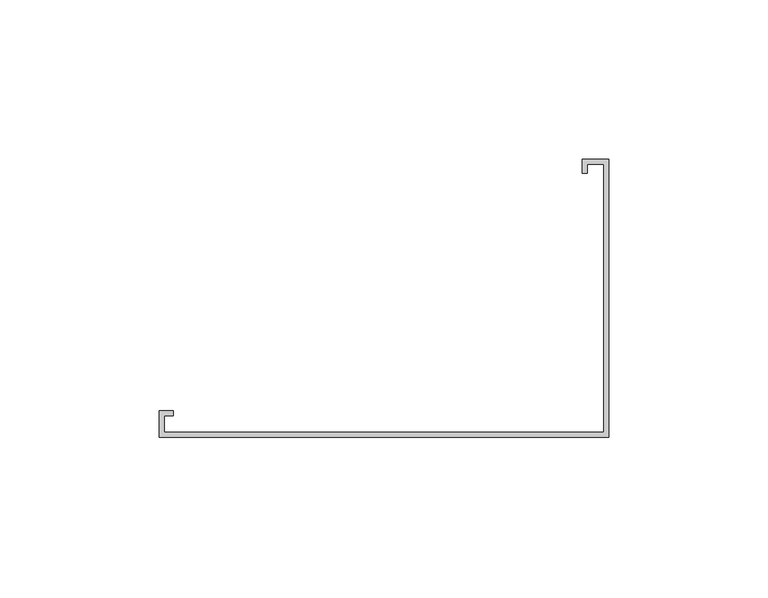
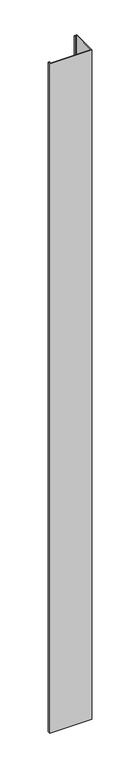
"""IFC4 building model written with IfcOpenShell, lengths in millimetres: proxy geometry, Generic Models 2:Generic Models 2:310765:Generic Models 2:310765 : Generic Models 2:Generic Models 2:310765:54 : Generic Models 2:Generic Models 2:310765:Generic Models 2:310765 : Generic Models 2:Generic Models 2:310765:300385."""

from ifc_helpers import new_model, si_unit, frame, origin, place, context, project, spatial, polyline, outline, extrude, source, transform, mapped, element, save


def generic_models_4d06f7c5(model_context):
    return source(origin(), model_context, "Body", "SweptSolid", [
        extrude(outline(polyline([(667632.8492598, -568190.3678931), (667641.2956314, -568190.3678931), (667641.2956314, -568277.8175782), (667499.9588141, -568277.8175782), (667499.9588141, -568269.3712067), (667504.3461407, -568269.3712067), (667504.3461407, -568270.9587067), (667501.5463141, -568270.9587067), (667501.5463141, -568276.2300782), (667639.7081314, -568276.2300782), (667639.7081314, -568191.9553931), (667634.4367598, -568191.9553931), (667634.4367598, -568194.7552197), (667632.8492598, -568194.7552197), (667632.8492598, -568190.3678931)])), frame((0.0, 0.0, 6165.85), z_axis=(0.0, 0.0, 1.0), x_axis=(1.0, 0.0, 0.0)), (0.0, 0.0, 1.0), 2389.9179991),
    ])


if __name__ == "__main__":
    model = new_model("IFC4")
    model_context = context("Model", 3, world=origin())
    ifc_project = project(units=[si_unit("LENGTHUNIT", "METRE", prefix="MILLI")], contexts=[model_context])
    site = spatial("IfcSite", under=ifc_project)
    building = spatial("IfcBuilding", under=site)
    placement = place(None, origin())
    generic_models_shape = generic_models_4d06f7c5(model_context)
    element("IfcBuildingElementProxy", 1, Name="Generic Models 2:Generic Models 2:310765:Generic Models 2:310765 : Generic Models 2:Generic Models 2:310765:54 : Generic Models 2:Generic Models 2:310765:Generic Models 2:310765 : Generic Models 2:Generic Models 2:310765:300385", ObjectType="Generic Models 2:Generic Models 2:310765:Generic Models 2:310765 : Generic Models 2:Generic Models 2:310765:54 : Generic Models 2:Generic Models 2:310765:Generic Models 2:310765 : Generic Models 2:Generic Models 2:310765:300385", at=placement, inside=building, context=model_context, shape_type="MappedRepresentation", body=[
        mapped(generic_models_shape, transform((0.0, 0.0, 0.0), x_axis=(1.0, 0.0, 0.0), y_axis=(0.0, 1.0, 0.0), z_axis=(0.0, 0.0, 1.0))),
    ])
    save(model, "model.ifc")

# Revit data of these elements
# Type "Generic Models 2:Generic Models 2:310765:Generic Models 2:310765 : Generic Models 2:Generic Models 2:310765:54 : Generic Models 2:Generic Models 2:310765:Generic Models 2:310765 : Generic Models 2:Generic Models 2:310765:300385"
#   NameOverride = "Generic Models 2:Generic Models 2:310765:Generic Models 2:310765 : Generic Models 2:Generic Models 2:310765:300385"
#   ObjectTypeOverride = "Generic Models 2:310765 : Generic Models 2:Generic Models 2:310765"
#   Reference = "Generic Models 2"
#   Tag = "300385"
# Element 1 (IfcBuildingElementProxy, "Generic Models 2:Generic Models 2:310765:Generic Models 2:310765 : Generic Models 2:Generic Models 2:310765:54 : Generic Models 2:Generic Models 2:310765:Generic Models 2:310765 : Generic Models 2:Generic Models 2:310765:300385")
#   Materials on its faces: "BRAKE METAL CLOSURE TRIM"
# Materials
#   "BRAKE METAL CLOSURE TRIM": class "Unassigned", colour RGB 210 209 208, transparency 0, Cost = 0
